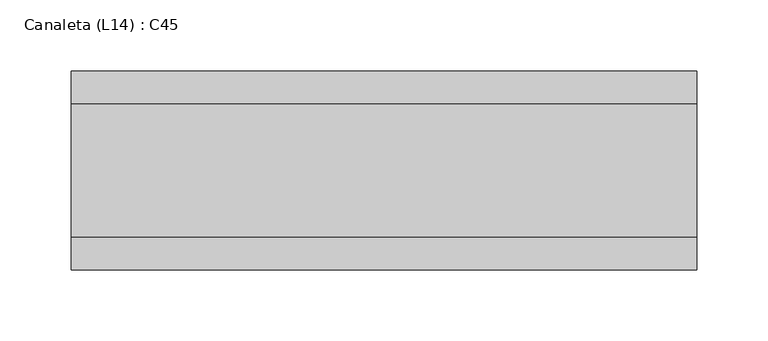
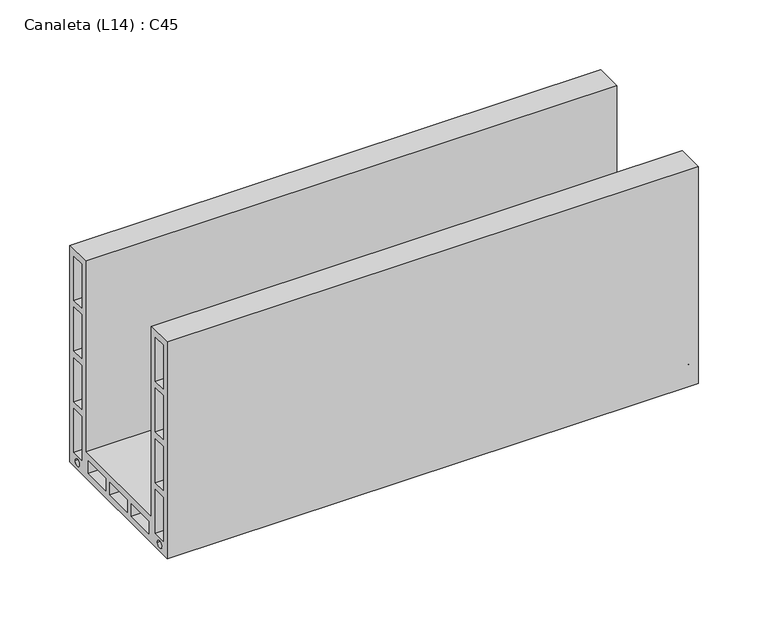
"""IFC4 building model written with IfcOpenShell, lengths in millimetres: proxy geometry, Canaleta (L14) : C45."""

from ifc_helpers import new_model, si_unit, point, frame, frame_2d, origin, place, context, project, spatial, polyline, circle_curve, trimmed, segment, composite_curve, outline, extrude, source, transform, mapped, element, save


def canaleta_l14_c45_20544c2f(model_context):
    return source(origin(), model_context, "Body", "SweptSolid", [
        extrude(outline(polyline([(-140.0, 0.0), (-140.0, 190.0), (-117.0, 190.0), (-117.0, 23.0), (-23.0, 23.0), (-23.0, 190.0), (0.0, 190.0), (0.0, 0.0), (-140.0, 0.0)]), holes=[polyline([(-123.0, 184.0), (-134.0, 184.0), (-134.0, 145.5), (-123.0, 145.5), (-123.0, 184.0)]), polyline([(-123.0, 139.5), (-134.0, 139.5), (-134.0, 101.0), (-123.0, 101.0), (-123.0, 139.5)]), polyline([(-123.0, 95.0), (-134.0, 95.0), (-134.0, 56.5), (-123.0, 56.5), (-123.0, 95.0)]), polyline([(-123.0, 50.5), (-134.0, 50.5), (-134.0, 12.0), (-123.0, 12.0), (-123.0, 50.5)]), composite_curve([segment(trimmed(circle_curve(frame_2d((-128.9426557, 6.2112346)), 3.0), [point((-125.9426557, 6.2112346))], [point((-131.9426557, 6.2112346))], True, "CARTESIAN"), True, "CONTINUOUS"), segment(trimmed(circle_curve(frame_2d((-128.9426557, 6.2112346)), 3.0), [point((-131.9426557, 6.2112346))], [point((-125.9426557, 6.2112346))], True, "CARTESIAN"), True, "CONTINUOUS")], self_intersect=False), polyline([(-17.0, 184.0), (-17.0, 145.5), (-6.0, 145.5), (-6.0, 184.0), (-17.0, 184.0)]), polyline([(-17.0, 139.5), (-17.0, 101.0), (-6.0, 101.0), (-6.0, 139.5), (-17.0, 139.5)]), polyline([(-17.0, 95.0), (-17.0, 56.5), (-6.0, 56.5), (-6.0, 95.0), (-17.0, 95.0)]), polyline([(-17.0, 50.5), (-17.0, 12.0), (-6.0, 12.0), (-6.0, 50.5), (-17.0, 50.5)]), composite_curve([segment(trimmed(circle_curve(frame_2d((-11.0573443, 6.2112346)), 3.0), [point((-8.0573443, 6.2112346))], [point((-14.0573443, 6.2112346))], True, "CARTESIAN"), True, "CONTINUOUS"), segment(trimmed(circle_curve(frame_2d((-11.0573443, 6.2112346)), 3.0), [point((-14.0573443, 6.2112346))], [point((-8.0573443, 6.2112346))], True, "CARTESIAN"), True, "CONTINUOUS")], self_intersect=False), polyline([(-88.5, 17.0), (-113.5, 17.0), (-113.5, 6.0), (-88.5, 6.0), (-88.5, 17.0)]), polyline([(-57.5, 17.0), (-82.5, 17.0), (-82.5, 6.0), (-57.5, 6.0), (-57.5, 17.0)]), polyline([(-26.5, 17.0), (-51.5, 17.0), (-51.5, 6.0), (-26.5, 6.0), (-26.5, 17.0)])]), frame((0.0, 0.0, 0.0), z_axis=(1.0, 0.0, 0.0), x_axis=(0.0, 1.0, 0.0)), (0.0, 0.0, 1.0), 440.0),
    ])


if __name__ == "__main__":
    model = new_model("IFC4")
    model_context = context("Model", 3, world=origin())
    ifc_project = project(units=[si_unit("LENGTHUNIT", "METRE", prefix="MILLI")], contexts=[model_context])
    site = spatial("IfcSite", under=ifc_project)
    building = spatial("IfcBuilding", under=site)
    placement = place(None, origin())
    canaleta_l14_c45_shape = canaleta_l14_c45_20544c2f(model_context)
    element("IfcBuildingElementProxy", 1, Name="Canaleta (L14) : C45", ObjectType="Canaleta (L14) : C45", at=placement, inside=building, context=model_context, shape_type="MappedRepresentation", body=[
        mapped(canaleta_l14_c45_shape, transform((0.0, 0.0, 0.0), x_axis=(1.0, 0.0, 0.0), y_axis=(0.0, 1.0, 0.0), z_axis=(0.0, 0.0, 1.0))),
    ])
    save(model, "model.ifc")

# Revit data of these elements
# Type "Canaleta (L14) : C45"
#   Comprimento = 0.440 m
#   Material [instance default] = Blocos Cerâmicos
#   Default Elevation = 0
# Element 1 (IfcBuildingElementProxy, "Canaleta (L14) : C45")
#   Materials on its faces: "Blocos Cerâmicos"
# Materials
#   "Blocos Cerâmicos": class "Genérico", colour RGB 177 84 47, transparency 0, Cost = 0
